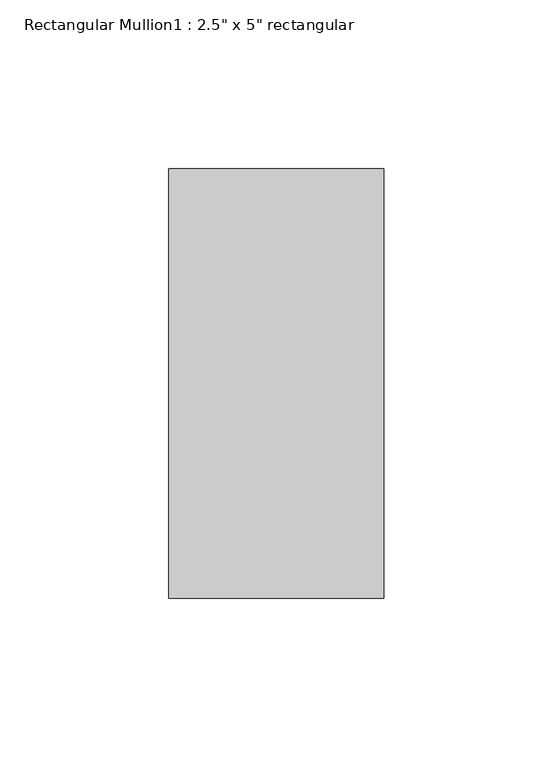
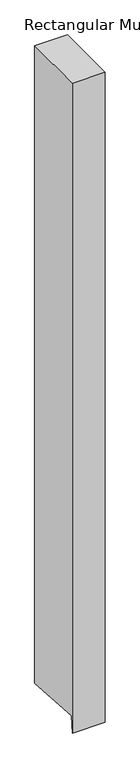
"""IFC4 building model written with IfcOpenShell, lengths in millimetres: member geometry."""

from ifc_helpers import new_model, si_unit, frame, origin, place, context, project, spatial, polyline, outline, extrude, source, transform, mapped, element, save


def member_1ee05d72(model_context):
    return source(origin(), model_context, "Body", "SweptSolid", [
        extrude(outline(polyline([(-63.5, 0.0), (63.5, 0.0), (63.5, -1307.2809876), (-61.0425175, -1298.2675313), (-63.5, -1332.2235469), (-63.5, 0.0)])), frame((-63.5, 0.0, 0.0), z_axis=(1.0, 0.0, 0.0), x_axis=(0.0, 1.0, 0.0)), (0.0, 0.0, 1.0), 63.5),
    ])


if __name__ == "__main__":
    model = new_model("IFC4")
    model_context = context("Model", 3, world=origin())
    ifc_project = project(units=[si_unit("LENGTHUNIT", "METRE", prefix="MILLI")], contexts=[model_context])
    site = spatial("IfcSite", under=ifc_project)
    building = spatial("IfcBuilding", under=site)
    placement = place(None, origin())
    member_shape = member_1ee05d72(model_context)
    element("IfcMember", 1, ObjectType="Rectangular Mullion1 : 2.5\" x 5\" rectangular", at=placement, inside=building, context=model_context, shape_type="MappedRepresentation", body=[
        mapped(member_shape, transform((0.0, 0.0, 0.0), x_axis=(1.0, 0.0, 0.0), y_axis=(0.0, 1.0, 0.0), z_axis=(0.0, 0.0, 1.0))),
    ])
    save(model, "model.ifc")

# Revit data of these elements
# Type "Rectangular Mullion1 : 2.5\" x 5\" rectangular"
#   built-in parameter 1007304 = 0.416667 (stored number, unit not read)
#   built-in parameter 1007301 = 0.104167 (stored number, unit not read)
#   built-in parameter 1007300 = 0.104167 (stored number, unit not read)
# Element 1 (IfcMember, "Rectangular Mullion1 : 2.5\" x 5\" rectangular")
#   Materials on its faces: "support-frame"
# Materials
#   "support-frame": class "Unassigned", colour RGB 233 233 233, transparency 0, Cost = 0
